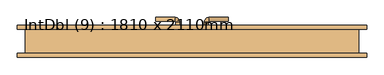
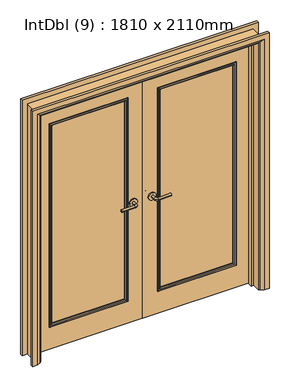
# IFC4 building model written with IfcOpenShell, lengths in millimetres: door geometry, IntDbl (9) : 1810 x 2110mm.
# Revit data of these elements (continued)
# Type "IntDbl (9) : 1810 x 2110mm" (continued)
#   Door Panel Offset = 0 mm
#   Structural Tolerance = 8 mm
#   Tolerance = 3 mm
#   UnderCut = 7 mm
#   Width = 1810 mm
#   Architrave Setback = 5 mm
#   Vis - Ironmongery = yes
#   Vis - Glazing Bars = yes
#   Material Ironmongery = Door - Handle
#   Material Glass = Door - Glazing
#   Material Frame = Door - Frame/Mullion
#   Material Door = Door - Panel
#   Material Beading = Door - Panel
#   Material Architrave = Door - Architrave
#   Function = (empty or 0)
#   Wall Closure = (empty or 0)
# Element 1 (IfcDoor, "IntDbl (9) : 1810 x 2110mm")
#   Materials on its faces: "Door - Panel", "Door - Handle", "Door - Architrave", "Door - Frame/Mullion", "Door - Glazing"
# Materials
#   "Door - Handle": class "Miscellaneous", colour RGB 0 0 0, transparency 0, Keynote = "P21"
#   "Door - Glazing": class "Miscellaneous", colour RGB 0 0 255, transparency 0.75
#   "Door - Frame/Mullion": class "Wood", colour RGB 212 179 113, transparency 0, Keynote = "L20"
#   "Door - Panel": class "Wood", colour RGB 210 159 95, transparency 0, Keynote = "L20"
#   "Door - Architrave": class "Wood", colour RGB 154 90 5, transparency 0, Keynote = "P20"
